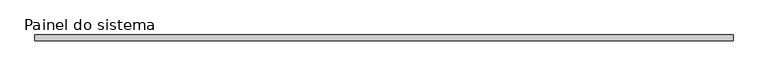
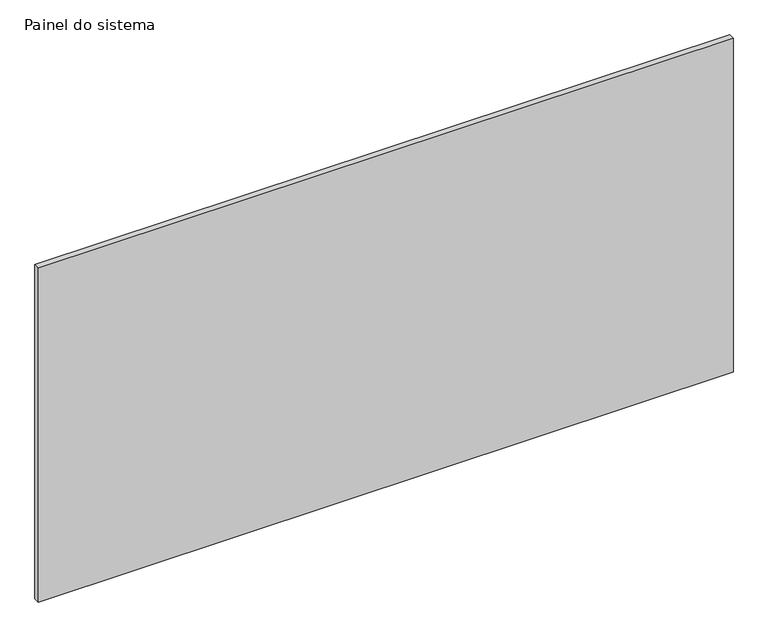
"""IFC4 building model written with IfcOpenShell, lengths in millimetres: plate geometry, Painel do sistema : Envidraçado."""

from ifc_helpers import new_model, si_unit, origin, origin_with_axes, place, context, project, spatial, polyline, outline, extrude, source, transform, mapped, element, save


def painel_do_sistema_5ef9eced(model_context):
    return source(origin(), model_context, "Body", "SweptSolid", [
        extrude(outline(polyline([(1475.0, 24.5), (-1475.0, 24.5), (-1475.0, 49.5), (1475.0, 49.5), (1475.0, 24.5)])), origin_with_axes(), (0.0, 0.0, 1.0), 1500.0),
    ])


if __name__ == "__main__":
    model = new_model("IFC4")
    model_context = context("Model", 3, world=origin())
    ifc_project = project(units=[si_unit("LENGTHUNIT", "METRE", prefix="MILLI")], contexts=[model_context])
    site = spatial("IfcSite", under=ifc_project)
    building = spatial("IfcBuilding", under=site)
    placement = place(None, origin())
    painel_do_sistema_shape = painel_do_sistema_5ef9eced(model_context)
    element("IfcPlate", 1, ObjectType="Painel do sistema : Envidraçado", at=placement, inside=building, context=model_context, shape_type="MappedRepresentation", body=[
        mapped(painel_do_sistema_shape, transform((0.0, 0.0, 0.0), x_axis=(1.0, 0.0, 0.0), y_axis=(0.0, 1.0, 0.0), z_axis=(0.0, 0.0, 1.0))),
    ])
    save(model, "model.ifc")

# Revit data of these elements
# Type "Painel do sistema : Envidraçado"
#   Construction Type Id = "GSP4R"
#   Analytic Construction = "Vidraça única Pilkington 1/8 pol"
#   Visual Light Transmittance = 0.9
#   Solar Heat Gain Coefficient = 0.86
#   Heat Transfer Coefficient (U) = 6.7069 W/(m²·K)
# Element 1 (IfcPlate, "Painel do sistema : Envidraçado")
#   Materials on its faces: "Vidro"
# Materials
#   "Vidro": class "Vidro", colour RGB 0 128 192, transparency 0.9, Description = "Vidro de sílica", Cost = 0
